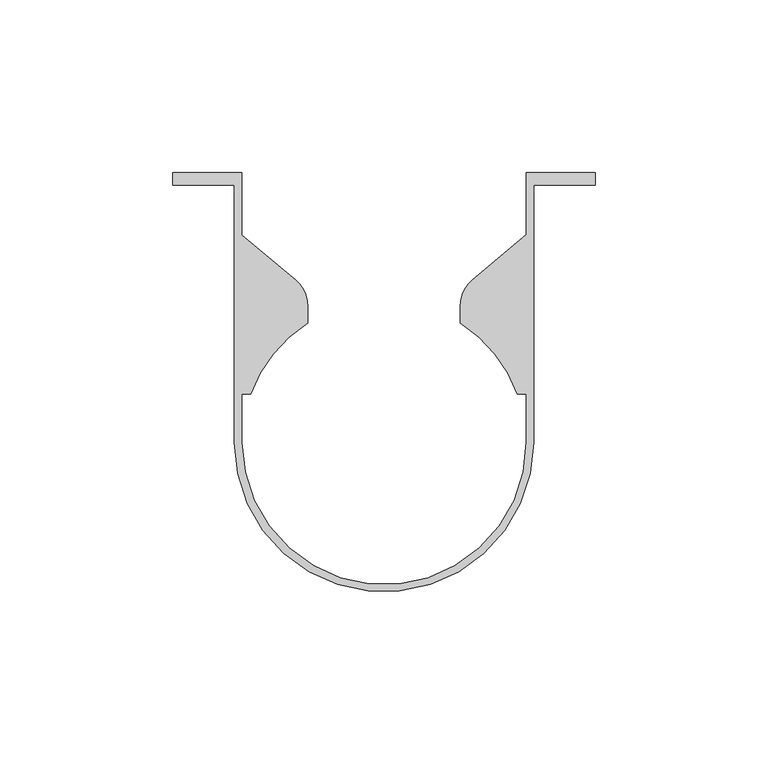
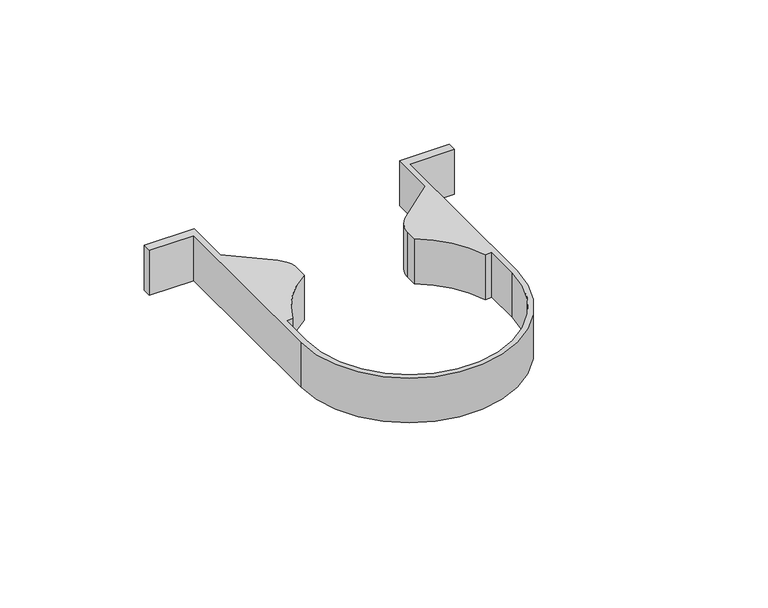
"""IFC4 building model written with IfcOpenShell, lengths in millimetres: proxy geometry, TN_ПВС 125-82_Хомут крепления трубы : TN_ПВС 125-82_Хомут крепления трубы."""

from ifc_helpers import new_model, si_unit, point, frame, frame_2d, origin, origin_2d, place, context, project, spatial, polyline, circle_curve, trimmed, segment, composite_curve, outline, extrude, source, transform, mapped, element, save


def generic_models_4e55d5ee(model_context):
    return source(origin(), model_context, "Body", "SweptSolid", [
        extrude(outline(composite_curve([segment(polyline([(41.1459233, 78.0), (61.0, 78.0), (61.0, 74.5), (43.2220121, 74.5), (43.2220121, 0.0)]), True, "CONTINUOUS"), segment(trimmed(circle_curve(frame_2d((-0.0424661, 0.1408408)), 43.2647075), [point((43.2220121, 0.0))], [point((-43.3069443, 0.0))], False, "CARTESIAN"), True, "CONTINUOUS"), segment(polyline([(-43.3069443, 0.0), (-43.3069443, 74.5), (-61.0, 74.5), (-61.0, 78.0), (-41.0540767, 78.0), (-41.0540767, 60.0453757), (-25.5721239, 47.0544749)]), True, "CONTINUOUS"), segment(trimmed(circle_curve(frame_2d((-32.0, 39.3940304)), 10.0), [point((-25.5721239, 47.0544749))], [point((-22.0, 39.3940304))], False, "CARTESIAN"), True, "CONTINUOUS"), segment(polyline([(-22.0, 39.3940304), (-22.0, 34.5976878)]), True, "CONTINUOUS"), segment(trimmed(circle_curve(origin_2d(), 41.0), [point((-22.0, 34.5976878))], [point((-38.5356977, 14.0))], True, "CARTESIAN"), True, "CONTINUOUS"), segment(polyline([(-38.5356977, 14.0), (-41.0540767, 14.0), (-41.0540767, 0.0)]), True, "CONTINUOUS"), segment(trimmed(circle_curve(frame_2d((0.0459233, 0.0)), 41.1), [point((-41.0540767, 0.0))], [point((41.1459233, 0.0))], True, "CARTESIAN"), True, "CONTINUOUS"), segment(polyline([(41.1459233, 0.0), (41.1459233, 14.0), (38.5356977, 14.0)]), True, "CONTINUOUS"), segment(trimmed(circle_curve(origin_2d(), 41.0), [point((38.5356977, 14.0))], [point((22.0, 34.5976878))], True, "CARTESIAN"), True, "CONTINUOUS"), segment(polyline([(22.0, 34.5976878), (22.0, 39.3940304)]), True, "CONTINUOUS"), segment(trimmed(circle_curve(frame_2d((32.0, 39.3940304)), 10.0), [point((22.0, 39.3940304))], [point((25.5721239, 47.0544749))], False, "CARTESIAN"), True, "CONTINUOUS"), segment(polyline([(25.5721239, 47.0544749), (41.1459233, 60.1224442), (41.1459233, 78.0)]), True, "CONTINUOUS")], self_intersect=False)), frame((0.0, 0.0, -9.5), z_axis=(0.0, 0.0, 1.0), x_axis=(1.0, 0.0, 0.0)), (0.0, 0.0, 1.0), 19.0),
    ])


if __name__ == "__main__":
    model = new_model("IFC4")
    model_context = context("Model", 3, world=origin())
    ifc_project = project(units=[si_unit("LENGTHUNIT", "METRE", prefix="MILLI")], contexts=[model_context])
    site = spatial("IfcSite", under=ifc_project)
    building = spatial("IfcBuilding", under=site)
    placement = place(None, origin())
    generic_models_shape = generic_models_4e55d5ee(model_context)
    element("IfcBuildingElementProxy", 1, Name="TN_ПВС 125-82_Хомут крепления трубы : TN_ПВС 125-82_Хомут крепления трубы", ObjectType="TN_ПВС 125-82_Хомут крепления трубы : TN_ПВС 125-82_Хомут крепления трубы", at=placement, inside=building, context=model_context, shape_type="MappedRepresentation", body=[
        mapped(generic_models_shape, transform((0.0, 0.0, 0.0), x_axis=(1.0, 0.0, 0.0), y_axis=(0.0, 1.0, 0.0), z_axis=(0.0, 0.0, 1.0))),
    ])
    save(model, "model.ifc")

# Revit data of these elements
# Type "TN_ПВС 125-82_Хомут крепления трубы : TN_ПВС 125-82_Хомут крепления трубы"
#   Description = "Предназначен для фиксации трубы к фасаду"
#   Manufacturer = "ТехноНИКОЛЬ"
#   Model = "Комплектующие к водосточным системам"
#   URL = "https://tn-vodostok.ru/catalog/pvh/"
#   ADSK_Обозначение = "ТехноНИКОЛЬ"
#   ADSK_Наименование краткое = "Хомут"
#   ADSK_Наименование = "Хомут крепления трубы"
#   ADSK_Масса_Текст = ""
#   ADSK_Марка = ""
#   ADSK_Код изделия = ""
#   ADSK_Завод-изготовитель = "ТехноНИКОЛЬ"
#   ADSK_Единица измерения = "шт."
#   ADSK_Группирование = "Комплектующие к водосточным системам"
#   ADSK_URL страницы изделия = "https://tn-vodostok.ru/catalog/pvh/"
#   ADSK_URL документации изделия = "https://tn-vodostok.ru/upload/iblock/c42/c427963cb77eb5c3c51f0cfb870e9e52.pdf"
#   ADSK_Размер_Ширина = 122 mm
#   ADSK_Размер_Длина = 121.121 mm
#   ADSK_Размер_Диаметр = 82.2 mm
#   ADSK_Размер_Высота = 19 mm
#   ADSK_Количество = 1
#   ADSK_Материал [instance default] = TN_Пластик_Коричневый_RAL8019
#   Default Elevation = 0
# Element 1 (IfcBuildingElementProxy, "TN_ПВС 125-82_Хомут крепления трубы : TN_ПВС 125-82_Хомут крепления трубы")
#   Materials on its faces: "TN_Пластик_Коричневый_RAL8019"
# Materials
#   "TN_Пластик_Коричневый_RAL8019": class "Типовые", colour RGB 61 54 53, transparency 0, Cost = 0
